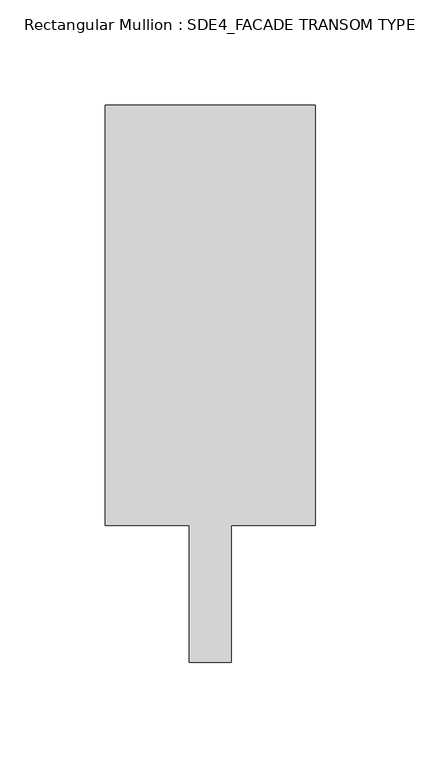
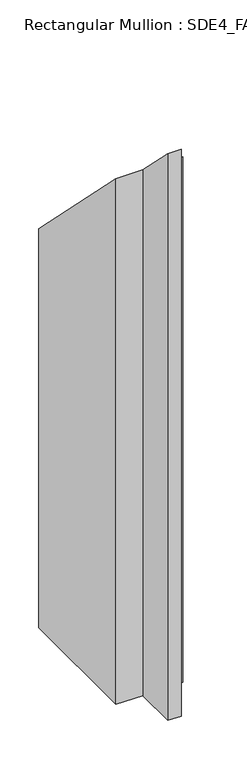
"""IFC4 building model written with IfcOpenShell, lengths in millimetres: member geometry, Rectangular Mullion : SDE4_FACADE TRANSOM TYPE 2."""

from ifc_helpers import new_model, si_unit, origin, place, context, project, spatial, faceted_brep, source, transform, mapped, element, save


def rectangular_mullion_sde4_facade_transom_type_2_f32353d7(model_context):
    return source(origin(), model_context, "Body", "Brep", [
        faceted_brep([(50.0, 132.5, -762.4189914), (50.0, -67.5, -762.4189914), (10.0, -67.5, -762.4189914), (10.0, -132.5, -762.4189914), (-10.0, -132.5, -762.4189914), (-10.0, -67.5, -762.4189914), (-50.0, -67.5, -762.4189914), (-50.0, 132.5, -762.4189914), (-50.0, 132.5, -132.5), (50.0, 132.5, -132.5), (-50.0, -67.5, 67.5), (-10.0, -67.5, 67.5), (-10.0, -132.5, 132.5), (10.0, -132.5, 132.5), (10.0, -67.5, 67.5), (50.0, -67.5, 67.5)], [[[0, 1, 2, 3, 4, 5, 6, 7]], [[8, 9, 0, 7]], [[10, 8, 7, 6]], [[11, 10, 6, 5]], [[12, 11, 5, 4]], [[13, 12, 4, 3]], [[14, 13, 3, 2]], [[15, 14, 2, 1]], [[9, 15, 1, 0]], [[9, 8, 10, 11, 12, 13, 14, 15]]]),
    ])


if __name__ == "__main__":
    model = new_model("IFC4")
    model_context = context("Model", 3, world=origin())
    ifc_project = project(units=[si_unit("LENGTHUNIT", "METRE", prefix="MILLI")], contexts=[model_context])
    site = spatial("IfcSite", under=ifc_project)
    building = spatial("IfcBuilding", under=site)
    placement = place(None, origin())
    rectangular_mullion_sde4_facade_transom_type_2_shape = rectangular_mullion_sde4_facade_transom_type_2_f32353d7(model_context)
    element("IfcMember", 1, ObjectType="Rectangular Mullion : SDE4_FACADE TRANSOM TYPE 2", at=placement, inside=building, context=model_context, shape_type="MappedRepresentation", body=[
        mapped(rectangular_mullion_sde4_facade_transom_type_2_shape, transform((0.0, 0.0, 0.0), x_axis=(1.0, 0.0, 0.0), y_axis=(0.0, 1.0, 0.0), z_axis=(0.0, 0.0, 1.0))),
    ])
    save(model, "model.ifc")

# Revit data of these elements
# Type "Rectangular Mullion : SDE4_FACADE TRANSOM TYPE 2"
#   built-in parameter 1007322 = 0.869423 (stored number, unit not read)
#   built-in parameter 1007321 = 0.164042 (stored number, unit not read)
#   built-in parameter 1007320 = 0.164042 (stored number, unit not read)
